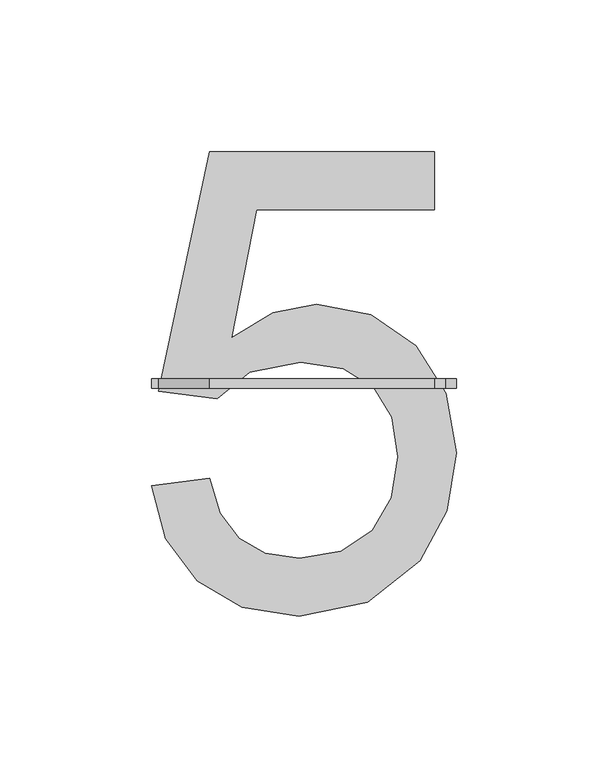
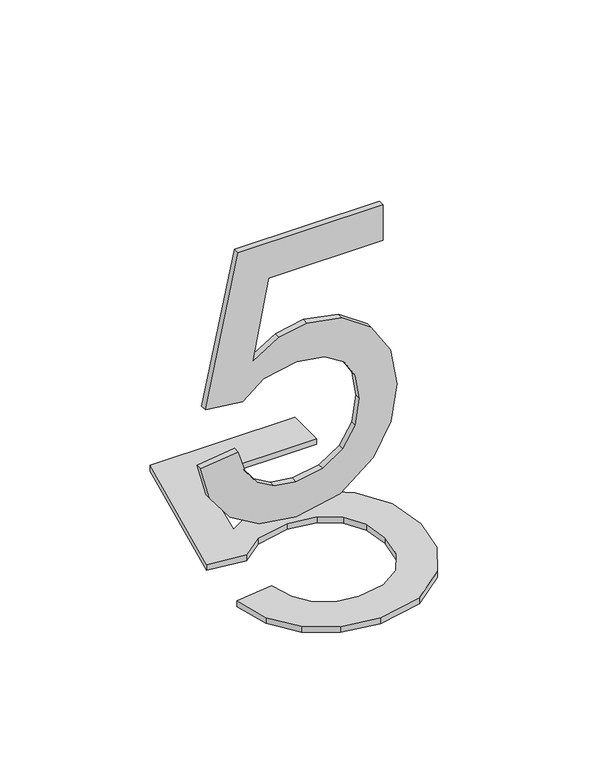
"""IFC4 building model written with IfcOpenShell, lengths in millimetres: proxy geometry, Grid Number1_FedEx : Grid Number1_FedEx."""

from ifc_helpers import new_model, si_unit, frame, origin, origin_with_axes, place, context, project, spatial, polyline, outline, extrude, source, transform, mapped, element, save


def entourage_38603b63(model_context):
    return source(origin(), model_context, "Body", "SweptSolid", [
        extrude(outline(polyline([(-157.1123024, 187.250035), (-137.9753753, 189.6421509), (-134.4619551, 178.1534537), (-128.3321581, 169.9258832), (-119.614017, 164.9781279), (-108.3355644, 163.3288761), (-94.6182749, 165.6228779), (-84.3396519, 172.5048832), (-77.9201847, 183.1806347), (-75.7803623, 196.8558753), (-77.7846938, 209.7321866), (-83.7976882, 219.5809762), (-93.8660666, 225.8322478), (-108.0365499, 227.916005), (-124.8374263, 224.5894689), (-135.5832594, 215.9554256), (-154.7201865, 218.3475415), (-137.9753753, 297.2873657), (-63.8197829, 297.2873657), (-63.8197829, 278.1504386), (-122.5013757, 278.1504386), (-130.6868972, 235.9893961), (-117.0163287, 244.2870481), (-102.691666, 247.0529321), (-84.8115342, 243.6236097), (-69.9682682, 233.3356426), (-59.9746435, 217.6560705), (-56.6434352, 198.0519333), (-59.6429243, 178.9150062), (-68.6413914, 162.5439631), (-85.8721012, 148.7799526), (-108.410318, 144.191949), (-127.2061817, 147.140045), (-142.1802665, 155.9843328), (-152.4448732, 169.6969502), (-157.1123024, 187.250035)])), origin_with_axes(), (0.0, 0.0, 1.0), 3.175),
        extrude(outline(polyline([(55.1458633, -157.1123024), (37.5927786, -152.4448732), (23.8801611, -142.1802665), (15.0358733, -127.2061817), (12.0877774, -108.410318), (16.6757809, -85.8721012), (30.4397914, -68.6413914), (46.8108345, -59.6429243), (65.9477616, -56.6434352), (85.5518988, -59.9746435), (101.2314709, -69.9682682), (111.5194381, -84.8115342), (114.9487604, -102.691666), (112.1828764, -117.0163287), (103.8852245, -130.6868972), (146.0462669, -122.5013757), (146.0462669, -63.8197829), (165.183194, -63.8197829), (165.183194, -137.9753753), (86.2433698, -154.7201865), (83.8512539, -135.5832594), (92.4852972, -124.8374263), (95.8118333, -108.0365499), (93.7280762, -93.8660666), (87.4768046, -83.7976882), (77.6280149, -77.7846938), (64.7517036, -75.7803623), (51.076463, -77.9201847), (40.4007115, -84.3396519), (33.5187062, -94.6182749), (31.2247044, -108.3355644), (32.8739562, -119.614017), (37.8217115, -128.3321581), (46.049282, -134.4619551), (57.5379792, -137.9753753), (55.1458633, -157.1123024)])), frame((0.0, 219.3456765, 0.0), z_axis=(0.0, 1.0, 0.0), x_axis=(0.0, 0.0, 1.0)), (0.0, 0.0, 1.0), 3.175),
    ])


if __name__ == "__main__":
    model = new_model("IFC4")
    model_context = context("Model", 3, world=origin())
    ifc_project = project(units=[si_unit("LENGTHUNIT", "METRE", prefix="MILLI")], contexts=[model_context])
    site = spatial("IfcSite", under=ifc_project)
    building = spatial("IfcBuilding", under=site)
    placement = place(None, origin())
    entourage_shape = entourage_38603b63(model_context)
    element("IfcBuildingElementProxy", 1, Name="Grid Number1_FedEx : Grid Number1_FedEx", ObjectType="Grid Number1_FedEx : Grid Number1_FedEx", at=placement, inside=building, context=model_context, shape_type="MappedRepresentation", body=[
        mapped(entourage_shape, transform((0.0, 0.0, 0.0), x_axis=(1.0, 0.0, 0.0), y_axis=(0.0, 1.0, 0.0), z_axis=(0.0, 0.0, 1.0))),
    ])
    save(model, "model.ifc")

# Revit data of these elements
# Type "Grid Number1_FedEx : Grid Number1_FedEx"
#   Grid [instance default] = "S.8"
#   Label Width [instance default] = 1' - 0"
#   Half Box Width2 [instance default] = 0' - 6.13846"
#   Half Box Width [instance default] = 0' - 6"
#   Robust [instance default] = yes
#   Height = 0
#   Assembly Code = ""
# Element 1 (IfcBuildingElementProxy, "Grid Number1_FedEx : Grid Number1_FedEx")
#   Grid = "5"
#   Robust = no
#   Materials on its faces: "Letter"
# Materials
#   "Letter": class "Unassigned", colour RGB 178 187 30, transparency 0, Comments = "Rendering appearance not upgraded "
